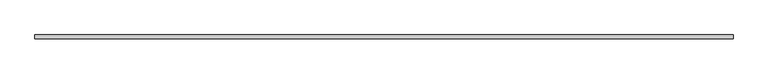
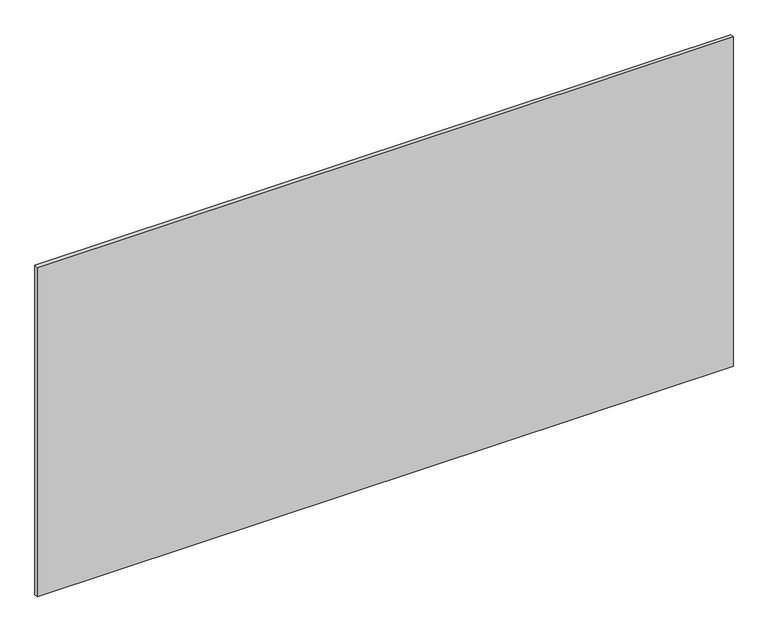
"""IFC4 building model written with IfcOpenShell, lengths in millimetres: proxy geometry, Inner panel:Inner panel:1:Inner panel:1 : Inner panel:Inner panel:300324:300043:Inner panel:1:Inner panel:1 : Inner panel:Inner panel:300324:300043 : Inner panel:Inner panel:1:Inner panel:1 : Inner panel:Inner panel:300324:300043:11 : Inner panel:Inner panel:1:Inner panel:1 : Inner panel:Inner panel:300324:300043:Inner panel:1:Inner panel:1 : Inner panel:Inner panel:300324:300043 : Inner panel:Inner panel:1:Inner panel:1 : Inner panel:Inner panel:300324:300043:300031."""

from ifc_helpers import new_model, si_unit, frame, origin, place, context, project, spatial, polyline, outline, extrude, source, transform, mapped, element, save


def generic_models_ed5fab44(model_context):
    return source(origin(), model_context, "Body", "SweptSolid", [
        extrude(outline(polyline([(568007.8867239, -579000.6913841), (570446.2867239, -579000.6913841), (570446.2867239, -579013.3913841), (568007.8867239, -579013.3913841), (568007.8867239, -579000.6913841)])), frame((0.0, 0.0, 4946.65), z_axis=(0.0, 0.0, 1.0), x_axis=(1.0, 0.0, 0.0)), (0.0, 0.0, 1.0), 1219.2),
    ])


if __name__ == "__main__":
    model = new_model("IFC4")
    model_context = context("Model", 3, world=origin())
    ifc_project = project(units=[si_unit("LENGTHUNIT", "METRE", prefix="MILLI")], contexts=[model_context])
    site = spatial("IfcSite", under=ifc_project)
    building = spatial("IfcBuilding", under=site)
    placement = place(None, origin())
    generic_models_shape = generic_models_ed5fab44(model_context)
    element("IfcBuildingElementProxy", 1, Name="Inner panel:Inner panel:1:Inner panel:1 : Inner panel:Inner panel:300324:300043:Inner panel:1:Inner panel:1 : Inner panel:Inner panel:300324:300043 : Inner panel:Inner panel:1:Inner panel:1 : Inner panel:Inner panel:300324:300043:11 : Inner panel:Inner panel:1:Inner panel:1 : Inner panel:Inner panel:300324:300043:Inner panel:1:Inner panel:1 : Inner panel:Inner panel:300324:300043 : Inner panel:Inner panel:1:Inner panel:1 : Inner panel:Inner panel:300324:300043:300031", ObjectType="Inner panel:Inner panel:1:Inner panel:1 : Inner panel:Inner panel:300324:300043:Inner panel:1:Inner panel:1 : Inner panel:Inner panel:300324:300043 : Inner panel:Inner panel:1:Inner panel:1 : Inner panel:Inner panel:300324:300043:11 : Inner panel:Inner panel:1:Inner panel:1 : Inner panel:Inner panel:300324:300043:Inner panel:1:Inner panel:1 : Inner panel:Inner panel:300324:300043 : Inner panel:Inner panel:1:Inner panel:1 : Inner panel:Inner panel:300324:300043:300031", at=placement, inside=building, context=model_context, shape_type="MappedRepresentation", body=[
        mapped(generic_models_shape, transform((0.0, 0.0, 0.0), x_axis=(1.0, 0.0, 0.0), y_axis=(0.0, 1.0, 0.0), z_axis=(0.0, 0.0, 1.0))),
    ])
    save(model, "model.ifc")

# Revit data of these elements
# Type "Inner panel:Inner panel:1:Inner panel:1 : Inner panel:Inner panel:300324:300043:Inner panel:1:Inner panel:1 : Inner panel:Inner panel:300324:300043 : Inner panel:Inner panel:1:Inner panel:1 : Inner panel:Inner panel:300324:300043:11 : Inner panel:Inner panel:1:Inner panel:1 : Inner panel:Inner panel:300324:300043:Inner panel:1:Inner panel:1 : Inner panel:Inner panel:300324:300043 : Inner panel:Inner panel:1:Inner panel:1 : Inner panel:Inner panel:300324:300043:300031"
#   NameOverride = "Inner panel:Inner panel:1:Inner panel:1 : Inner panel:Inner panel:300324:300043:Inner panel:1:Inner panel:1 : Inner panel:Inner panel:300324:300043 : Inner panel:Inner panel:1:Inner panel:1 : Inner panel:Inner panel:300324:300043:300031"
#   ObjectTypeOverride = "Inner panel:1:Inner panel:1 : Inner panel:Inner panel:300324:300043 : Inner panel:Inner panel:1:Inner panel:1 : Inner panel:Inner panel:300324:300043"
#   Reference = "Inner panel"
#   Tag = "300031"
# Element 1 (IfcBuildingElementProxy, "Inner panel:Inner panel:1:Inner panel:1 : Inner panel:Inner panel:300324:300043:Inner panel:1:Inner panel:1 : Inner panel:Inner panel:300324:300043 : Inner panel:Inner panel:1:Inner panel:1 : Inner panel:Inner panel:300324:300043:11 : Inner panel:Inner panel:1:Inner panel:1 : Inner panel:Inner panel:300324:300043:Inner panel:1:Inner panel:1 : Inner panel:Inner panel:300324:300043 : Inner panel:Inner panel:1:Inner panel:1 : Inner panel:Inner panel:300324:300043:300031")
#   Materials on its faces: "1/2\" FIBERGLASS MAT GYPSUM PANELS"
# Materials
#   "1/2\" FIBERGLASS MAT GYPSUM PANELS": class "Generic", colour RGB 171 170 168, transparency 0, Description = "Gypsum Wall Board", Cost = 0
